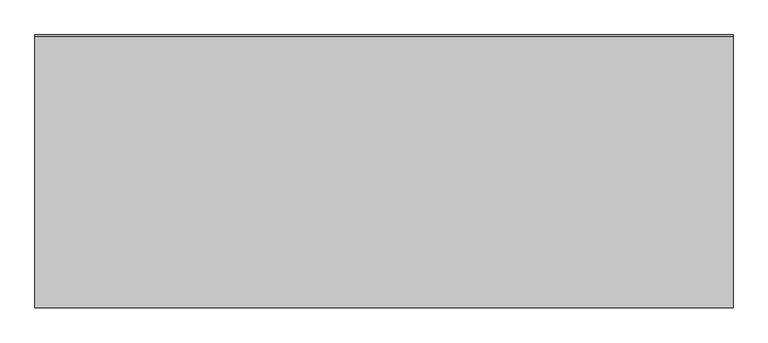
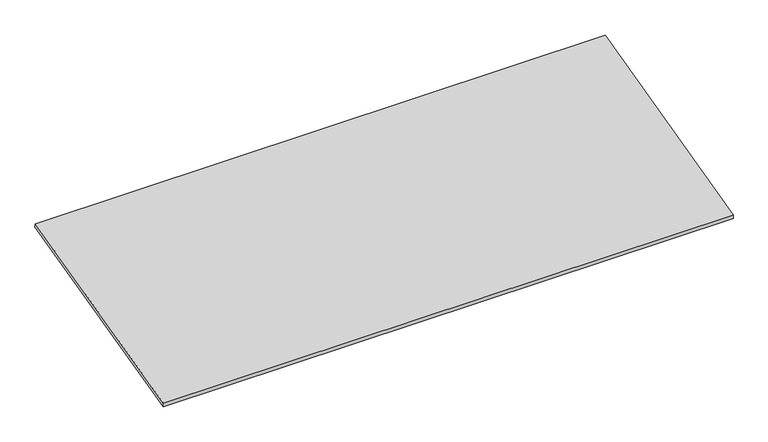
"""IFC4 building model written with IfcOpenShell, lengths in millimetres: proxy geometry, Roof001 1014 : Roof001 1014."""

from ifc_helpers import new_model, si_unit, frame, origin, place, context, project, spatial, polyline, outline, extrude, source, transform, mapped, element, save


def generic_models_f9485631(model_context):
    return source(origin(), model_context, "Body", "SweptSolid", [
        extrude(outline(polyline([(9636.2273859, 43625.0361034), (9639.5003656, 43611.9531504), (8857.5938813, 43416.342571), (8857.5938813, 43430.3777272), (9636.2273859, 43625.0361034)])), frame((3694.2883192, 0.0, 0.0), z_axis=(1.0, 0.0, 0.0), x_axis=(0.0, 1.0, 0.0)), (0.0, 0.0, 1.0), 2000.0),
    ])


if __name__ == "__main__":
    model = new_model("IFC4")
    model_context = context("Model", 3, world=origin())
    ifc_project = project(units=[si_unit("LENGTHUNIT", "METRE", prefix="MILLI")], contexts=[model_context])
    site = spatial("IfcSite", under=ifc_project)
    building = spatial("IfcBuilding", under=site)
    placement = place(None, origin())
    generic_models_shape = generic_models_f9485631(model_context)
    element("IfcBuildingElementProxy", 1, Name="Roof001 1014 : Roof001 1014", ObjectType="Roof001 1014 : Roof001 1014", at=placement, inside=building, context=model_context, shape_type="MappedRepresentation", body=[
        mapped(generic_models_shape, transform((0.0, 0.0, 0.0), x_axis=(1.0, 0.0, 0.0), y_axis=(0.0, 1.0, 0.0), z_axis=(0.0, 0.0, 1.0))),
    ])
    save(model, "model.ifc")

# Revit data of these elements
# Type "Roof001 1014 : Roof001 1014"
#   NameOverride = "Roof001"
# Element 1 (IfcBuildingElementProxy, "Roof001 1014 : Roof001 1014")
#   Materials on its faces: "STANDING SEAM METAL ROOF"
# Materials
#   "STANDING SEAM METAL ROOF": class "Unassigned", colour RGB 128 128 128, transparency 0
